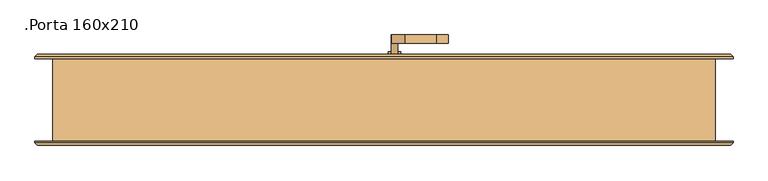
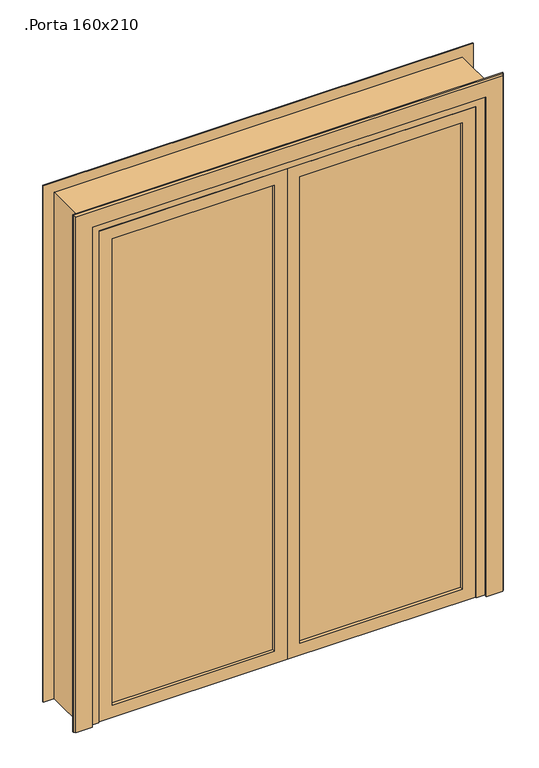
"""IFC4 building model written with IfcOpenShell, lengths in millimetres: door geometry, Abertura da porta e vidraça com revestimento : .Porta 160x210."""

from ifc_helpers import new_model, si_unit, point, frame, frame_2d, origin, place, context, project, spatial, polyline, circle_curve, trimmed, segment, composite_curve, outline, extrude, faceted_brep, source, transform, mapped, element, save


def porta_160x210_6cb1d5fe(model_context):
    return source(origin(), model_context, "Body", "SolidModel", [
        extrude(outline(polyline([(-680.0, -7.0), (-680.0, 7.0), (-50.0, 7.0), (-50.0, -7.0), (-680.0, -7.0)])), frame((0.0, 0.0, 50.0), z_axis=(0.0, 0.0, 1.0), x_axis=(1.0, 0.0, 0.0)), (0.0, 0.0, 1.0), 1930.0),
        extrude(outline(polyline([(2030.0, -730.0), (0.0, -730.0), (0.0, 0.0), (2030.0, 0.0), (2030.0, -730.0)]), holes=[polyline([(50.0, -680.0), (1980.0, -680.0), (1980.0, -50.0), (50.0, -50.0), (50.0, -680.0)])]), frame((0.0, -20.0, 0.0), z_axis=(0.0, 1.0, 0.0), x_axis=(0.0, 0.0, 1.0)), (0.0, 0.0, 1.0), 40.0),
        extrude(outline(polyline([(680.0, -7.0), (50.0, -7.0), (50.0, 7.0), (680.0, 7.0), (680.0, -7.0)])), frame((0.0, 0.0, 50.0), z_axis=(0.0, 0.0, 1.0), x_axis=(1.0, 0.0, 0.0)), (0.0, 0.0, 1.0), 1930.0),
        extrude(outline(polyline([(2030.0, 730.0), (2030.0, 0.0), (0.0, 0.0), (0.0, 730.0), (2030.0, 730.0)]), holes=[polyline([(50.0, 680.0), (50.0, 50.0), (1980.0, 50.0), (1980.0, 680.0), (50.0, 680.0)])]), frame((0.0, -20.0, 0.0), z_axis=(0.0, 1.0, 0.0), x_axis=(0.0, 0.0, 1.0)), (0.0, 0.0, 1.0), 40.0),
        extrude(outline(polyline([(-50.0, 89.0), (-50.0, 65.0), (-687.0, 65.0), (-687.0, 89.0), (-50.0, 89.0)])), frame((0.0, 0.0, 53.0), z_axis=(0.0, 0.0, 1.0), x_axis=(1.0, 0.0, 0.0)), (0.0, 0.0, 1.0), 1934.0),
        extrude(outline(polyline([(2037.0, -737.0), (3.0, -737.0), (3.0, 0.0), (2037.0, 0.0), (2037.0, -737.0)]), holes=[polyline([(53.0, -687.0), (1987.0, -687.0), (1987.0, -50.0), (53.0, -50.0), (53.0, -687.0)])]), frame((0.0, 57.0, 0.0), z_axis=(0.0, 1.0, 0.0), x_axis=(0.0, 0.0, 1.0)), (0.0, 0.0, 1.0), 40.0),
        extrude(outline(composite_curve([segment(trimmed(circle_curve(frame_2d((840.0, 25.0)), 15.0), [point((840.0, 40.0))], [point((840.0, 10.0))], False, "CARTESIAN"), True, "CONTINUOUS"), segment(trimmed(circle_curve(frame_2d((840.0, 25.0)), 15.0), [point((840.0, 10.0))], [point((840.0, 40.0))], False, "CARTESIAN"), True, "CONTINUOUS")], self_intersect=False)), frame((0.0, 107.0, 0.0), z_axis=(0.0, 1.0, 0.0), x_axis=(0.0, 0.0, 1.0)), (0.0, 0.0, 1.0), 10.0),
        extrude(outline(composite_curve([segment(trimmed(circle_curve(frame_2d((840.0, 25.0)), 15.0), [point((840.0, 40.0))], [point((840.0, 10.0))], False, "CARTESIAN"), True, "CONTINUOUS"), segment(trimmed(circle_curve(frame_2d((840.0, 25.0)), 15.0), [point((840.0, 10.0))], [point((840.0, 40.0))], False, "CARTESIAN"), True, "CONTINUOUS")], self_intersect=False)), frame((0.0, 37.0, 0.0), z_axis=(0.0, 1.0, 0.0), x_axis=(0.0, 0.0, 1.0)), (0.0, 0.0, 1.0), 10.0),
        extrude(outline(composite_curve([segment(trimmed(circle_curve(frame_2d((900.0, 25.0)), 8.0), [point((904.6523287, 18.4918637))], [point((900.0, 33.0))], False, "CARTESIAN"), True, "CONTINUOUS"), segment(trimmed(circle_curve(frame_2d((894.8738613, 50.3861901)), 18.1261387), [point((900.0, 33.0))], [point((913.0, 50.3861901))], True, "CARTESIAN"), True, "CONTINUOUS"), segment(polyline([(913.0, 50.3861901), (913.0, 126.6435909)]), True, "CONTINUOUS"), segment(trimmed(circle_curve(frame_2d((972.2709207, 123.0603388)), 59.3791355), [point((913.0, 126.6435909))], [point((922.2135558, 155.0))], False, "CARTESIAN"), True, "CONTINUOUS"), segment(polyline([(922.2135558, 155.0), (925.0, 155.0)]), True, "CONTINUOUS"), segment(trimmed(circle_curve(frame_2d((1003.2850638, 126.5772091)), 83.2850902), [point((925.0, 155.0))], [point((920.0, 126.6435909))], True, "CARTESIAN"), True, "CONTINUOUS"), segment(polyline([(920.0, 126.6435909), (920.0, 50.3674333)]), True, "CONTINUOUS"), segment(trimmed(circle_curve(frame_2d((882.7555521, 48.6675129)), 37.2832219), [point((920.0, 50.3674333))], [point((904.6523287, 18.4918637))], False, "CARTESIAN"), True, "CONTINUOUS")], self_intersect=False)), frame((0.0, 137.0, 0.0), z_axis=(0.0, 1.0, 0.0), x_axis=(0.0, 0.0, 1.0)), (0.0, 0.0, 1.0), 20.0),
        extrude(outline(composite_curve([segment(trimmed(circle_curve(frame_2d((894.8738682, 50.3861878)), 18.1261318), [point((899.9999903, 33.0))], [point((913.0, 50.3861878))], True, "CARTESIAN"), True, "CONTINUOUS"), segment(polyline([(913.0, 50.3861878), (913.0, 126.6435909)]), True, "CONTINUOUS"), segment(trimmed(circle_curve(frame_2d((972.2709207, 123.0603388)), 59.3791355), [point((913.0, 126.6435909))], [point((922.2135558, 155.0))], False, "CARTESIAN"), True, "CONTINUOUS"), segment(polyline([(922.2135558, 155.0), (925.0, 155.0)]), True, "CONTINUOUS"), segment(trimmed(circle_curve(frame_2d((1003.2850638, 126.5772091)), 83.2850902), [point((925.0, 155.0))], [point((920.0, 126.6435909))], True, "CARTESIAN"), True, "CONTINUOUS"), segment(polyline([(920.0, 126.6435909), (920.0, 50.3674333)]), True, "CONTINUOUS"), segment(trimmed(circle_curve(frame_2d((882.7555521, 48.6675129)), 37.2832219), [point((920.0, 50.3674333))], [point((904.6523287, 18.4918637))], False, "CARTESIAN"), True, "CONTINUOUS"), segment(trimmed(circle_curve(frame_2d((900.0, 25.0)), 8.0), [point((904.6523287, 18.4918637))], [point((899.9999903, 33.0))], False, "CARTESIAN"), True, "CONTINUOUS")], self_intersect=False)), frame((0.0, -3.0, 0.0), z_axis=(0.0, 1.0, 0.0), x_axis=(0.0, 0.0, 1.0)), (0.0, 0.0, 1.0), 20.0),
        extrude(outline(composite_curve([segment(trimmed(circle_curve(frame_2d((900.0, 25.0)), 8.0), [point((900.0, 33.0))], [point((900.0, 17.0))], False, "CARTESIAN"), True, "CONTINUOUS"), segment(trimmed(circle_curve(frame_2d((900.0, 25.0)), 8.0), [point((900.0, 17.0))], [point((900.0, 33.0))], False, "CARTESIAN"), True, "CONTINUOUS")], self_intersect=False)), frame((0.0, 107.0, 0.0), z_axis=(0.0, 1.0, 0.0), x_axis=(0.0, 0.0, 1.0)), (0.0, 0.0, 1.0), 30.0),
        extrude(outline(composite_curve([segment(trimmed(circle_curve(frame_2d((900.0, 25.0)), 8.0), [point((900.0, 33.0))], [point((900.0, 17.0))], False, "CARTESIAN"), True, "CONTINUOUS"), segment(trimmed(circle_curve(frame_2d((900.0, 25.0)), 8.0), [point((900.0, 17.0))], [point((900.0, 33.0))], False, "CARTESIAN"), True, "CONTINUOUS")], self_intersect=False)), frame((0.0, 17.0, 0.0), z_axis=(0.0, 1.0, 0.0), x_axis=(0.0, 0.0, 1.0)), (0.0, 0.0, 1.0), 30.0),
        extrude(outline(composite_curve([segment(trimmed(circle_curve(frame_2d((830.0, 25.0)), 25.0), [point((830.0, 0.0))], [point((830.0, 50.0))], False, "CARTESIAN"), True, "CONTINUOUS"), segment(polyline([(830.0, 50.0), (900.0, 50.0)]), True, "CONTINUOUS"), segment(trimmed(circle_curve(frame_2d((900.0, 25.0)), 25.0), [point((900.0, 50.0))], [point((900.0, 0.0))], False, "CARTESIAN"), True, "CONTINUOUS"), segment(polyline([(900.0, 0.0), (830.0, 0.0)]), True, "CONTINUOUS")], self_intersect=False)), frame((0.0, 97.0, 0.0), z_axis=(0.0, 1.0, 0.0), x_axis=(0.0, 0.0, 1.0)), (0.0, 0.0, 1.0), 10.0),
        extrude(outline(composite_curve([segment(trimmed(circle_curve(frame_2d((830.0, 25.0)), 25.0), [point((830.0, 0.0))], [point((830.0, 50.0))], False, "CARTESIAN"), True, "CONTINUOUS"), segment(polyline([(830.0, 50.0), (900.0, 50.0)]), True, "CONTINUOUS"), segment(trimmed(circle_curve(frame_2d((900.0, 25.0)), 25.0), [point((900.0, 50.0))], [point((900.0, 0.0))], False, "CARTESIAN"), True, "CONTINUOUS"), segment(polyline([(900.0, 0.0), (830.0, 0.0)]), True, "CONTINUOUS")], self_intersect=False)), frame((0.0, 47.0, 0.0), z_axis=(0.0, 1.0, 0.0), x_axis=(0.0, 0.0, 1.0)), (0.0, 0.0, 1.0), 10.0),
        extrude(outline(polyline([(50.0, 89.0), (687.0, 89.0), (687.0, 65.0), (50.0, 65.0), (50.0, 89.0)])), frame((0.0, 0.0, 53.0), z_axis=(0.0, 0.0, 1.0), x_axis=(1.0, 0.0, 0.0)), (0.0, 0.0, 1.0), 1934.0),
        extrude(outline(polyline([(2037.0, 737.0), (2037.0, 0.0), (3.0, 0.0), (3.0, 737.0), (2037.0, 737.0)]), holes=[polyline([(53.0, 687.0), (53.0, 50.0), (1987.0, 50.0), (1987.0, 687.0), (53.0, 687.0)])]), frame((0.0, 57.0, 0.0), z_axis=(0.0, 1.0, 0.0), x_axis=(0.0, 0.0, 1.0)), (0.0, 0.0, 1.0), 40.0),
        extrude(outline(polyline([(-50.0, -84.0), (-687.0, -84.0), (-687.0, -70.0), (-50.0, -70.0), (-50.0, -84.0)])), frame((0.0, 0.0, 53.0), z_axis=(0.0, 0.0, 1.0), x_axis=(1.0, 0.0, 0.0)), (0.0, 0.0, 1.0), 1934.0),
        extrude(outline(polyline([(3.0, -737.0), (3.0, 0.0), (2037.0, 0.0), (2037.0, -737.0), (3.0, -737.0)]), holes=[polyline([(1987.0, -687.0), (1987.0, -50.0), (53.0, -50.0), (53.0, -687.0), (1987.0, -687.0)])]), frame((0.0, -97.0, 0.0), z_axis=(0.0, 1.0, 0.0), x_axis=(0.0, 0.0, 1.0)), (0.0, 0.0, 1.0), 40.0),
        extrude(outline(polyline([(50.0, -84.0), (50.0, -70.0), (687.0, -70.0), (687.0, -84.0), (50.0, -84.0)])), frame((0.0, 0.0, 53.0), z_axis=(0.0, 0.0, 1.0), x_axis=(1.0, 0.0, 0.0)), (0.0, 0.0, 1.0), 1934.0),
        extrude(outline(polyline([(3.0, 737.0), (2037.0, 737.0), (2037.0, 0.0), (3.0, 0.0), (3.0, 737.0)]), holes=[polyline([(1987.0, 687.0), (53.0, 687.0), (53.0, 50.0), (1987.0, 50.0), (1987.0, 687.0)])]), frame((0.0, -97.0, 0.0), z_axis=(0.0, 1.0, 0.0), x_axis=(0.0, 0.0, 1.0)), (0.0, 0.0, 1.0), 40.0),
        faceted_brep([(-740.0, -100.0, 0.0), (-800.0, -100.0, 0.0), (-800.0, 100.0, 0.0), (-740.0, 100.0, 0.0), (-740.0, 54.0, 0.0), (-730.0, 54.0, 0.0), (-730.0, -54.0, 0.0), (-740.0, -54.0, 0.0), (-740.0, -100.0, 2040.0), (740.0, -100.0, 2040.0), (740.0, -100.0, 0.0), (800.0, -100.0, 0.0), (800.0, -100.0, 2100.0), (-800.0, -100.0, 2100.0), (-800.0, 100.0, 2100.0), (800.0, 100.0, 2100.0), (800.0, 100.0, 0.0), (740.0, 100.0, 0.0), (740.0, 100.0, 2040.0), (-740.0, 100.0, 2040.0), (-740.0, 54.0, 2040.0), (740.0, 54.0, 2040.0), (740.0, 54.0, 0.0), (730.0, 54.0, 0.0), (730.0, 54.0, 2030.0), (-730.0, 54.0, 2030.0), (-730.0, -54.0, 2030.0), (730.0, -54.0, 2030.0), (730.0, -54.0, 0.0), (740.0, -54.0, 0.0), (740.0, -54.0, 2040.0), (-740.0, -54.0, 2040.0)], [[[0, 1, 2, 3, 4, 5, 6, 7]], [[1, 0, 8, 9, 10, 11, 12, 13]], [[2, 1, 13, 14]], [[3, 2, 14, 15, 16, 17, 18, 19]], [[4, 3, 19, 20]], [[5, 4, 20, 21, 22, 23, 24, 25]], [[6, 5, 25, 26]], [[7, 6, 26, 27, 28, 29, 30, 31]], [[0, 7, 31, 8]], [[10, 29, 28, 23, 22, 17, 16, 11]], [[9, 30, 29, 10]], [[27, 24, 23, 28]], [[21, 18, 17, 22]], [[15, 12, 11, 16]], [[14, 13, 12, 15]], [[20, 19, 18, 21]], [[26, 25, 24, 27]], [[8, 31, 30, 9]]]),
        faceted_brep([(843.0, -104.0, 0.0), (837.0, -110.0, 0.0), (773.0, -110.0, 0.0), (773.0, -100.0, 0.0), (843.0, -100.0, 0.0), (843.0, -104.0, 2143.0), (837.0, -110.0, 2137.0), (-837.0, -110.0, 2137.0), (-837.0, -110.0, 0.0), (-773.0, -110.0, 0.0), (-773.0, -110.0, 2073.0), (773.0, -110.0, 2073.0), (773.0, -100.0, 2073.0), (-773.0, -100.0, 2073.0), (-773.0, -100.0, 0.0), (-843.0, -100.0, 0.0), (-843.0, -100.0, 2143.0), (843.0, -100.0, 2143.0), (-843.0, -104.0, 0.0), (-843.0, -104.0, 2143.0)], [[[0, 1, 2, 3, 4]], [[1, 0, 5, 6]], [[2, 1, 6, 7, 8, 9, 10, 11]], [[3, 2, 11, 12]], [[4, 3, 12, 13, 14, 15, 16, 17]], [[0, 4, 17, 5]], [[18, 15, 14, 9, 8]], [[19, 16, 15, 18]], [[13, 10, 9, 14]], [[7, 19, 18, 8]], [[6, 5, 19, 7]], [[12, 11, 10, 13]], [[5, 17, 16, 19]]]),
        faceted_brep([(843.0, 104.0, 0.0), (843.0, 100.0, 0.0), (773.0, 100.0, 0.0), (773.0, 110.0, 0.0), (837.0, 110.0, 0.0), (843.0, 104.0, 2143.0), (843.0, 100.0, 2143.0), (-843.0, 100.0, 2143.0), (-843.0, 100.0, 0.0), (-773.0, 100.0, 0.0), (-773.0, 100.0, 2073.0), (773.0, 100.0, 2073.0), (773.0, 110.0, 2073.0), (-773.0, 110.0, 2073.0), (-773.0, 110.0, 0.0), (-837.0, 110.0, 0.0), (-837.0, 110.0, 2137.0), (837.0, 110.0, 2137.0), (-843.0, 104.0, 0.0), (-843.0, 104.0, 2143.0)], [[[0, 1, 2, 3, 4]], [[1, 0, 5, 6]], [[2, 1, 6, 7, 8, 9, 10, 11]], [[3, 2, 11, 12]], [[4, 3, 12, 13, 14, 15, 16, 17]], [[0, 4, 17, 5]], [[18, 15, 14, 9, 8]], [[19, 16, 15, 18]], [[13, 10, 9, 14]], [[7, 19, 18, 8]], [[6, 5, 19, 7]], [[12, 11, 10, 13]], [[5, 17, 16, 19]]]),
    ])


if __name__ == "__main__":
    model = new_model("IFC4")
    model_context = context("Model", 3, world=origin())
    ifc_project = project(units=[si_unit("LENGTHUNIT", "METRE", prefix="MILLI")], contexts=[model_context])
    site = spatial("IfcSite", under=ifc_project)
    building = spatial("IfcBuilding", under=site)
    placement = place(None, origin())
    porta_160x210_shape = porta_160x210_6cb1d5fe(model_context)
    element("IfcDoor", 1, ObjectType="Abertura da porta e vidraça com revestimento : .Porta 160x210", at=placement, inside=building, context=model_context, shape_type="MappedRepresentation", body=[
        mapped(porta_160x210_shape, transform((0.0, 0.0, 0.0), x_axis=(1.0, 0.0, 0.0), y_axis=(0.0, 1.0, 0.0), z_axis=(0.0, 0.0, 1.0))),
    ])
    save(model, "model.ifc")

# Revit data of these elements
# Type "Abertura da porta e vidraça com revestimento : .Porta 160x210"
#   Type Mark = "50"
#   Construction Type Id = "MDOOR"
#   Analytic Construction = "Metal"
#   W1 = 0.046 m
#   Largura da apara = 0.07 m
#   Espessura da apara = 0.01 m
#   Rough Width = 1.60 m
#   Rough Height = 2.10 m
#   Largura da moldura do painel = 0.05 m
#   Espessura da moldura do painel = 0.04 m
#   Heat Transfer Coefficient (U) = 3.7021 W/(m²·K)
#   Height = 2.10 m
#   Width = 1.60 m
#   Largura da estrutura = 0.05 m
#   Define Thermal Properties by = 1
#   Function = 1
#   Material da apara = Aço inoxidável
#   Material do painel = Vidro
#   Material do puxador = Aço inoxidável
#   Vidro = Vidro
#   Material da moldura = Aço inoxidável
#   Visual Light Transmittance = 0
#   Solar Heat Gain Coefficient = 0
#   Wall Closure = (empty or 0)
# Element 1 (IfcDoor, "Abertura da porta e vidraça com revestimento : .Porta 160x210")
#   Materials on its faces: "Aço inoxidável", "Vidro"
# Materials
#   "Aço inoxidável": class "Metal", colour RGB 0 0 0, transparency 0, Description = "Aço inoxidável 18/8", Cost = 0
#   "Vidro": class "Vidro", colour RGB 0 128 192, transparency 0.9, Description = "Vidro de sílica", Cost = 0
